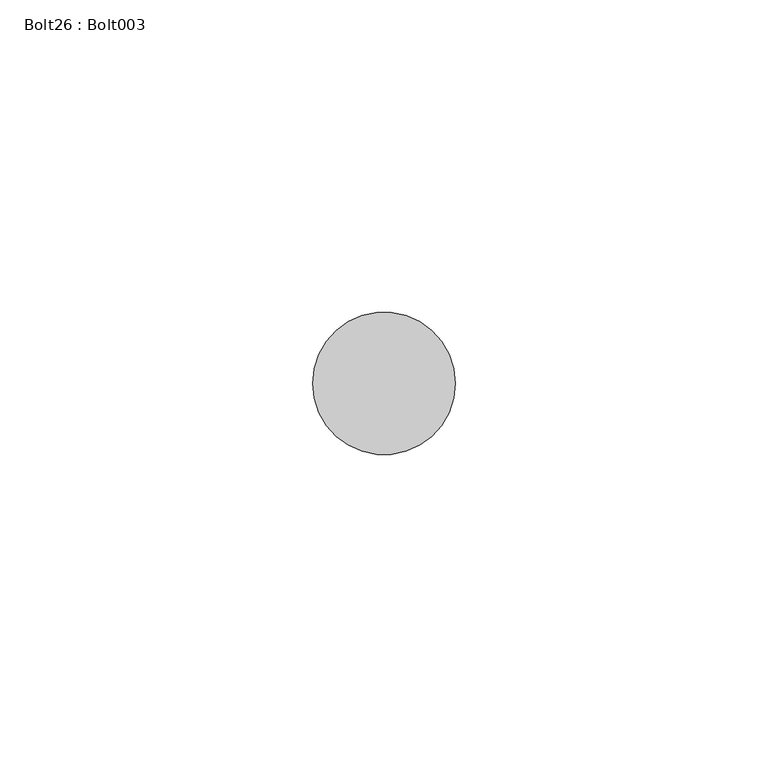
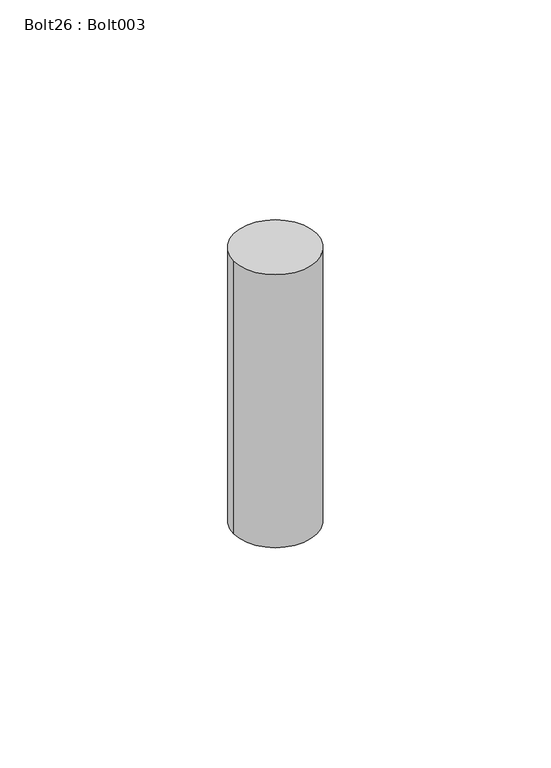
"""IFC4 building model written with IfcOpenShell, lengths in millimetres: proxy geometry, Bolt26 : Bolt003."""

from ifc_helpers import new_model, si_unit, point, frame, frame_2d, origin, place, context, project, spatial, circle_curve, trimmed, segment, composite_curve, outline, extrude, source, transform, mapped, element, save


def bolt26_bolt003_c467bee4(model_context):
    return source(origin(), model_context, "Body", "SweptSolid", [
        extrude(outline(composite_curve([segment(trimmed(circle_curve(frame_2d((5172.3828124, 1896.5882072)), 11.4045168), [point((5160.9782956, 1896.5882072))], [point((5183.7873292, 1896.5882072))], False, "CARTESIAN"), True, "CONTINUOUS"), segment(trimmed(circle_curve(frame_2d((5172.3828124, 1896.5882072)), 11.4045168), [point((5183.7873292, 1896.5882072))], [point((5160.9782956, 1896.5882072))], False, "CARTESIAN"), True, "CONTINUOUS")], self_intersect=False)), frame((0.0, 0.0, 36645.5959962), z_axis=(0.0, 0.0, 1.0), x_axis=(1.0, 0.0, 0.0)), (0.0, 0.0, 1.0), 79.375),
    ])


if __name__ == "__main__":
    model = new_model("IFC4")
    model_context = context("Model", 3, world=origin())
    ifc_project = project(units=[si_unit("LENGTHUNIT", "METRE", prefix="MILLI")], contexts=[model_context])
    site = spatial("IfcSite", under=ifc_project)
    building = spatial("IfcBuilding", under=site)
    placement = place(None, origin())
    bolt26_bolt003_shape = bolt26_bolt003_c467bee4(model_context)
    element("IfcBuildingElementProxy", 1, Name="Bolt26 : Bolt003", ObjectType="Bolt26 : Bolt003", at=placement, inside=building, context=model_context, shape_type="MappedRepresentation", body=[
        mapped(bolt26_bolt003_shape, transform((0.0, 0.0, 0.0), x_axis=(1.0, 0.0, 0.0), y_axis=(0.0, 1.0, 0.0), z_axis=(0.0, 0.0, 1.0))),
    ])
    save(model, "model.ifc")

# Revit data of these elements
# Type "Bolt26 : Bolt003"
#   NameOverride = "Bolt003"
# Element 1 (IfcBuildingElementProxy, "Bolt26 : Bolt003")
#   Materials on its faces: "STEEL ANGLE AND ANCHOR BOLT (SEE STRUCT. DWGS)"
# Materials
#   "STEEL ANGLE AND ANCHOR BOLT (SEE STRUCT. DWGS)": class "Unassigned", colour RGB 128 128 128, transparency 0, Cost = 0
